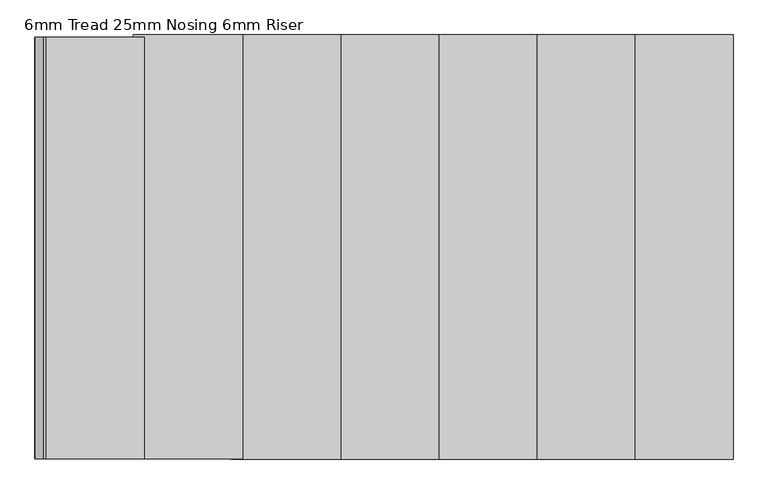
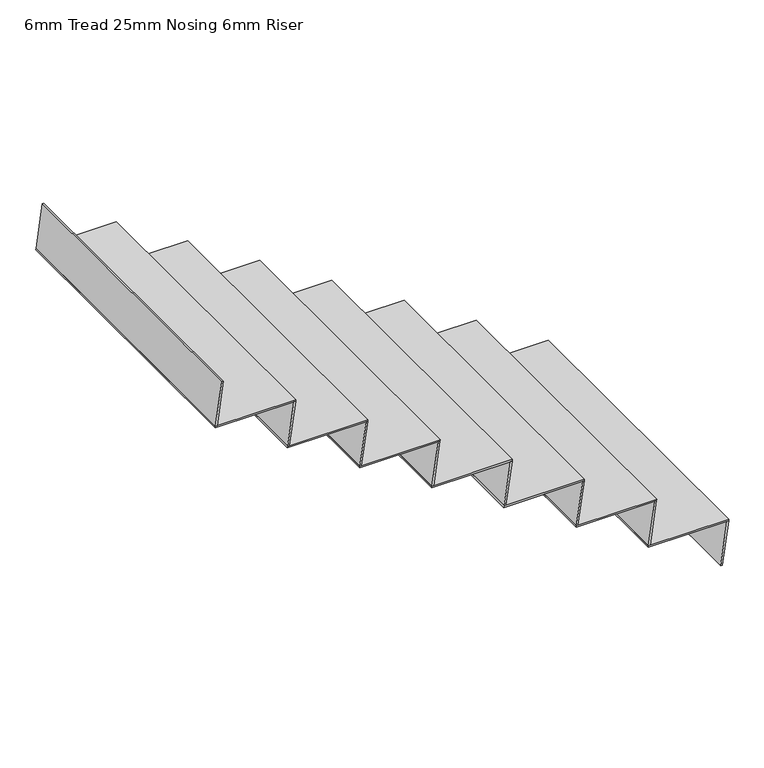
"""IFC4 building model written with IfcOpenShell, lengths in millimetres: stair flight geometry, 6mm Tread 25mm Nosing 6mm Riser."""

from ifc_helpers import new_model, si_unit, frame, origin, place, context, project, spatial, polyline, outline, extrude, source, transform, mapped, element, save


def stair_flight_6mm_tread_25mm_nosing_6mm_riser_c971a7fb(model_context):
    return source(origin(), model_context, "Body", "SweptSolid", [
        extrude(outline(polyline([(30764.7058824, 16350.0), (30764.7058824, 16043.9400908), (30758.7058824, 16043.0900908), (30758.7058824, 16349.15), (30764.7058824, 16350.0)])), frame((0.0, 12030.4345331, 0.0), z_axis=(0.0, 1.0, 0.0), x_axis=(0.0, 0.0, 1.0)), (0.0, 0.0, 1.0), 1190.0),
        extrude(outline(polyline([(30758.7058824, 16349.15), (30758.7058824, 16343.0900908), (30588.2352941, 16318.9400908), (30588.2352941, 16325.0), (30758.7058824, 16349.15)])), frame((0.0, 12030.4345331, 0.0), z_axis=(0.0, 1.0, 0.0), x_axis=(0.0, 0.0, 1.0)), (0.0, 0.0, 1.0), 1190.0),
        extrude(outline(polyline([(30935.1764706, 16074.15), (30935.1764706, 16068.0900908), (30764.7058824, 16043.9400908), (30764.7058824, 16050.0), (30935.1764706, 16074.15)])), frame((0.0, 12030.4345331, 0.0), z_axis=(0.0, 1.0, 0.0), x_axis=(0.0, 0.0, 1.0)), (0.0, 0.0, 1.0), 1190.0),
        extrude(outline(polyline([(30941.1764706, 16075.0), (30941.1764706, 15768.9400908), (30935.1764706, 15768.0900908), (30935.1764706, 16074.15), (30941.1764706, 16075.0)])), frame((0.0, 12030.4345331, 0.0), z_axis=(0.0, 1.0, 0.0), x_axis=(0.0, 0.0, 1.0)), (0.0, 0.0, 1.0), 1190.0),
        extrude(outline(polyline([(31111.6470588, 15799.15), (31111.6470588, 15793.0900908), (30941.1764706, 15768.9400908), (30941.1764706, 15775.0), (31111.6470588, 15799.15)])), frame((0.0, 12030.4345331, 0.0), z_axis=(0.0, 1.0, 0.0), x_axis=(0.0, 0.0, 1.0)), (0.0, 0.0, 1.0), 1190.0),
        extrude(outline(polyline([(31117.6470588, 15800.0), (31117.6470588, 15493.9400908), (31111.6470588, 15493.0900908), (31111.6470588, 15799.15), (31117.6470588, 15800.0)])), frame((0.0, 12030.4345331, 0.0), z_axis=(0.0, 1.0, 0.0), x_axis=(0.0, 0.0, 1.0)), (0.0, 0.0, 1.0), 1190.0),
        extrude(outline(polyline([(31288.1176471, 15524.15), (31288.1176471, 15518.0900908), (31117.6470588, 15493.9400908), (31117.6470588, 15500.0), (31288.1176471, 15524.15)])), frame((0.0, 12030.4345331, 0.0), z_axis=(0.0, 1.0, 0.0), x_axis=(0.0, 0.0, 1.0)), (0.0, 0.0, 1.0), 1190.0),
        extrude(outline(polyline([(31294.1176471, 15525.0), (31294.1176471, 15218.9400908), (31288.1176471, 15218.0900908), (31288.1176471, 15524.15), (31294.1176471, 15525.0)])), frame((0.0, 12030.4345331, 0.0), z_axis=(0.0, 1.0, 0.0), x_axis=(0.0, 0.0, 1.0)), (0.0, 0.0, 1.0), 1190.0),
        extrude(outline(polyline([(31464.5882353, 15249.15), (31464.5882353, 15243.0900908), (31294.1176471, 15218.9400908), (31294.1176471, 15225.0), (31464.5882353, 15249.15)])), frame((0.0, 12030.4345331, 0.0), z_axis=(0.0, 1.0, 0.0), x_axis=(0.0, 0.0, 1.0)), (0.0, 0.0, 1.0), 1190.0),
        extrude(outline(polyline([(31470.5882353, 15250.0), (31470.5882353, 14943.9400908), (31464.5882353, 14943.0900908), (31464.5882353, 15249.15), (31470.5882353, 15250.0)])), frame((0.0, 12030.4345331, 0.0), z_axis=(0.0, 1.0, 0.0), x_axis=(0.0, 0.0, 1.0)), (0.0, 0.0, 1.0), 1190.0),
        extrude(outline(polyline([(31641.0588235, 14974.15), (31641.0588235, 14968.0900908), (31470.5882353, 14943.9400908), (31470.5882353, 14950.0), (31641.0588235, 14974.15)])), frame((0.0, 12030.4345331, 0.0), z_axis=(0.0, 1.0, 0.0), x_axis=(0.0, 0.0, 1.0)), (0.0, 0.0, 1.0), 1190.0),
        extrude(outline(polyline([(31647.0588235, 14975.0), (31647.0588235, 14668.9400908), (31641.0588235, 14668.0900908), (31641.0588235, 14974.15), (31647.0588235, 14975.0)])), frame((0.0, 12030.4345331, 0.0), z_axis=(0.0, 1.0, 0.0), x_axis=(0.0, 0.0, 1.0)), (0.0, 0.0, 1.0), 1190.0),
        extrude(outline(polyline([(31994.0, 14424.15), (31994.0, 14418.0900908), (31823.5294118, 14393.9400908), (31823.5294118, 14400.0), (31994.0, 14424.15)])), frame((0.0, 12030.4345331, 0.0), z_axis=(0.0, 1.0, 0.0), x_axis=(0.0, 0.0, 1.0)), (0.0, 0.0, 1.0), 1184.0),
        extrude(outline(polyline([(31817.5294118, 14699.15), (31817.5294118, 14693.0900908), (31647.0588235, 14668.9400908), (31647.0588235, 14675.0), (31817.5294118, 14699.15)])), frame((0.0, 12030.4345331, 0.0), z_axis=(0.0, 1.0, 0.0), x_axis=(0.0, 0.0, 1.0)), (0.0, 0.0, 1.0), 1184.0),
        extrude(outline(polyline([(31823.5294118, 14700.0), (31823.5294118, 14393.9400908), (31817.5294118, 14393.0900908), (31817.5294118, 14699.15), (31823.5294118, 14700.0)])), frame((0.0, 12030.4345331, 0.0), z_axis=(0.0, 1.0, 0.0), x_axis=(0.0, 0.0, 1.0)), (0.0, 0.0, 1.0), 1184.0),
    ])


if __name__ == "__main__":
    model = new_model("IFC4")
    model_context = context("Model", 3, world=origin())
    ifc_project = project(units=[si_unit("LENGTHUNIT", "METRE", prefix="MILLI")], contexts=[model_context])
    site = spatial("IfcSite", under=ifc_project)
    building = spatial("IfcBuilding", under=site)
    placement = place(None, origin())
    stair_flight_6mm_tread_25mm_nosing_6mm_riser_shape = stair_flight_6mm_tread_25mm_nosing_6mm_riser_c971a7fb(model_context)
    element("IfcStairFlight", 1, ObjectType="6mm Tread 25mm Nosing 6mm Riser", at=placement, inside=building, context=model_context, shape_type="MappedRepresentation", body=[
        mapped(stair_flight_6mm_tread_25mm_nosing_6mm_riser_shape, transform((0.0, 0.0, 0.0), x_axis=(1.0, 0.0, 0.0), y_axis=(0.0, 1.0, 0.0), z_axis=(0.0, 0.0, 1.0))),
    ])
    save(model, "model.ifc")

# Revit data of these elements
# Element 1 (IfcStairFlight, "6mm Tread 25mm Nosing 6mm Riser")
#   Materials on its faces: "Steel, Paint Finish, Dark Gray"
# Materials
#   "Steel, Paint Finish, Dark Gray": class "Metal", colour RGB 89 89 89, transparency 0, Description = "Steel, paint finish, dark gray, glossy", Cost = 0
